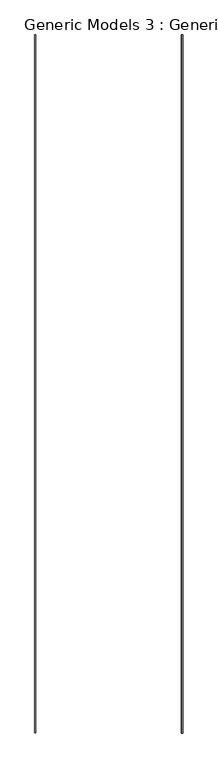
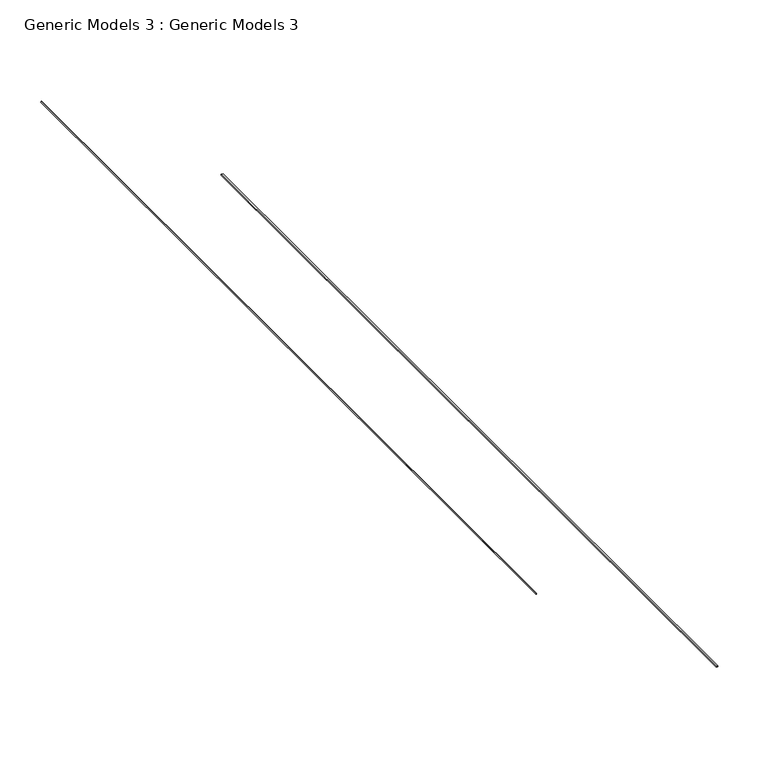
"""IFC4 building model written with IfcOpenShell, lengths in millimetres: proxy geometry, Generic Models 3 : Generic Models 3."""

from ifc_helpers import new_model, si_unit, frame, origin, place, context, project, spatial, polyline, outline, extrude, source, transform, mapped, element, save


def generic_models_3_generic_models_3_ad3143c0(model_context):
    return source(origin(), model_context, "Body", "SweptSolid", [
        extrude(outline(polyline([(0.0, -1208.478541), (0.0, 0.0), (1.0, 0.0), (1.0, -1208.478541), (0.0, -1208.478541)])), frame((22018.8034617, -8904.678541, 1722.3633882), z_axis=(0.07574648693489495, 0.0, 0.9971271081045896), x_axis=(-0.9971271081045896, 0.0, 0.07574648693489495)), (0.0, 0.0, 1.0), 1.7777373),
        extrude(outline(polyline([(0.0, -1208.8), (0.0, 0.0), (2.54, 0.0), (2.54, -1208.8), (0.0, -1208.8)])), frame((22274.3479268, -8905.0, 1525.1402282), z_axis=(0.07574648693490242, 0.0, 0.997127108104589), x_axis=(-0.997127108104589, 0.0, 0.07574648693490242)), (0.0, 0.0, 1.0), 1.1780051),
    ])


if __name__ == "__main__":
    model = new_model("IFC4")
    model_context = context("Model", 3, world=origin())
    ifc_project = project(units=[si_unit("LENGTHUNIT", "METRE", prefix="MILLI")], contexts=[model_context])
    site = spatial("IfcSite", under=ifc_project)
    building = spatial("IfcBuilding", under=site)
    placement = place(None, origin())
    generic_models_3_generic_models_3_shape = generic_models_3_generic_models_3_ad3143c0(model_context)
    element("IfcBuildingElementProxy", 1, Name="Generic Models 3 : Generic Models 3", ObjectType="Generic Models 3 : Generic Models 3", at=placement, inside=building, context=model_context, shape_type="MappedRepresentation", body=[
        mapped(generic_models_3_generic_models_3_shape, transform((0.0, 0.0, 0.0), x_axis=(1.0, 0.0, 0.0), y_axis=(0.0, 1.0, 0.0), z_axis=(0.0, 0.0, 1.0))),
    ])
    save(model, "model.ifc")

# Revit data of these elements
# Element 1 (IfcBuildingElementProxy, "Generic Models 3 : Generic Models 3")
#   Materials on its faces: "light mat"
# Materials
#   "light mat": class "Generic", colour RGB 120 120 120, transparency 0, Cost = 0
